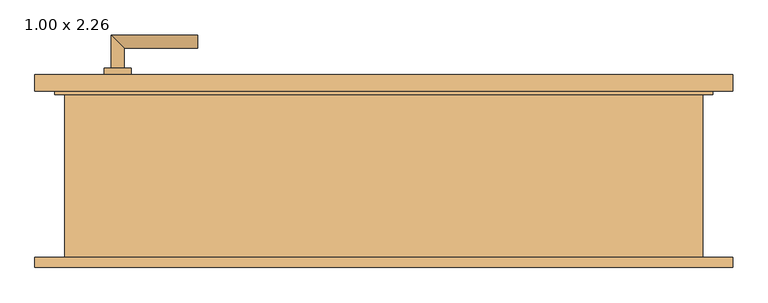
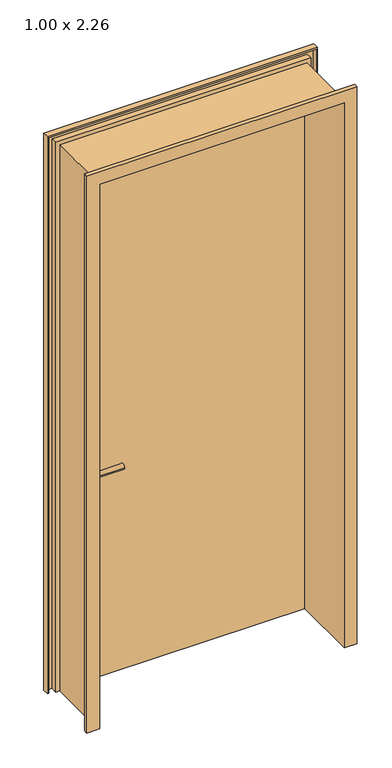
"""IFC4 building model written with IfcOpenShell, lengths in millimetres: door geometry, Drehflügel 1-flg - Stahlzarge : 1.00 x 2.26."""

import ifcopenshell
import ifcopenshell.guid

model = None  # the IFC model being written
_history = None  # IfcOwnerHistory: only IFC2X3 demands one
_inside = {}  # id of a spatial element -> (the spatial element, [elements in it])
_under = {}  # id of a project, library or spatial element -> (it, [spatial elements below it])
_declared = {}  # id of a project -> (the project, [libraries it declares])
_typed = {}  # id of a type object -> (the type object, [elements of that type])
_made_of = {}  # id of a material, layer set ... -> (it, [elements and type objects made of it])


def new_model(schema):
    """Start an empty IFC model of exactly this schema.

    Asked for "IFC4X3", IfcOpenShell would pick the latest addendum, in which some entities
    have other attributes; the version numbers below select the first issue.
    IFC2X3 requires an IfcOwnerHistory on every rooted entity: one is made here for all.
    """
    global model, _history
    if schema == "IFC4X3":
        model = ifcopenshell.file(schema_version=(4, 3, 0, 0))
    else:
        model = ifcopenshell.file(schema=schema)
    _inside.clear()
    _under.clear()
    _declared.clear()
    _typed.clear()
    _made_of.clear()
    _history = None
    if model.schema == "IFC2X3":
        org = make("IfcOrganization", Name="unknown")
        user = make(
            "IfcPersonAndOrganization",
            ThePerson=make("IfcPerson", FamilyName="unknown"),
            TheOrganization=org,
        )
        app = make(
            "IfcApplication",
            ApplicationDeveloper=org,
            Version="unknown",
            ApplicationFullName="unknown",
            ApplicationIdentifier="unknown",
        )
        _history = make(
            "IfcOwnerHistory",
            OwningUser=user,
            OwningApplication=app,
            ChangeAction="ADDED",
            CreationDate=0,
        )
    return model


def make(cls, **values):
    """One entity of the class cls with the attributes given. An attribute that is None is left unset."""
    return model.create_entity(
        cls, **{name: value for name, value in values.items() if value is not None}
    )


def rooted(cls, **values):
    """An entity with a GlobalId (a new one), such as an element, a storey or a relation."""
    return make(cls, GlobalId=ifcopenshell.guid.new(), OwnerHistory=_history, **values)


def si_unit(unit_type, name, prefix=None):
    """IfcSIUnit, for example si_unit("LENGTHUNIT", "METRE", prefix="MILLI")."""
    return make("IfcSIUnit", UnitType=unit_type, Prefix=prefix, Name=name)


def assignment(units):
    """IfcUnitAssignment: the units of a project."""
    return None if units is None else make("IfcUnitAssignment", Units=units)


def point(xyz):
    """IfcCartesianPoint."""
    return None if xyz is None else make("IfcCartesianPoint", Coordinates=xyz)


def direction(xyz):
    """IfcDirection."""
    return None if xyz is None else make("IfcDirection", DirectionRatios=xyz)


def frame(location, z_axis=None, x_axis=None):
    """IfcAxis2Placement3D, a coordinate frame: its origin and axes. An axis left out is left unset."""
    return make(
        "IfcAxis2Placement3D",
        Location=point(location),
        Axis=direction(z_axis),
        RefDirection=direction(x_axis),
    )


def frame_2d(location, x_axis=None):
    """IfcAxis2Placement2D, a coordinate frame in the plane: its origin and x axis."""
    return make(
        "IfcAxis2Placement2D", Location=point(location), RefDirection=direction(x_axis)
    )


def origin():
    """The frame at (0, 0, 0) with its axes left unset."""
    return frame((0.0, 0.0, 0.0))


def place(relative_to, where):
    """IfcLocalPlacement: puts the frame where relative to a parent placement (None: the world)."""
    return make(
        "IfcLocalPlacement", PlacementRelTo=relative_to, RelativePlacement=where
    )


def context(
    kind, dimensions, precision=None, world=None, true_north=None, identifier=None
):
    """IfcGeometricRepresentationContext, for example the 3D "Model" context."""
    return make(
        "IfcGeometricRepresentationContext",
        ContextIdentifier=identifier,
        ContextType=kind,
        CoordinateSpaceDimension=dimensions,
        Precision=precision,
        WorldCoordinateSystem=world,
        TrueNorth=true_north,
    )


def project(units=None, contexts=None):
    """IfcProject with its units and contexts."""
    return rooted(
        "IfcProject",
        Name="project",
        RepresentationContexts=contexts,
        UnitsInContext=assignment(units),
    )


def spatial(cls, under=None, at=None, **own):
    """A site, building, storey or space (cls), placed at a placement, below another one or the project."""
    s = rooted(cls, ObjectPlacement=at, **own)
    if under is not None:
        _under.setdefault(under.id(), (under, []))[1].append(s)
    return s


def polyline(points):
    """IfcPolyline through the points."""
    return make("IfcPolyline", Points=[point(p) for p in points])


def circle_curve(where, radius):
    """IfcCircle in the frame where."""
    return make("IfcCircle", Position=where, Radius=radius)


def ellipse_curve(where, semi_axis1, semi_axis2):
    """IfcEllipse in the frame where."""
    return make(
        "IfcEllipse", Position=where, SemiAxis1=semi_axis1, SemiAxis2=semi_axis2
    )


def trimmed(basis, trim1, trim2, sense, master):
    """IfcTrimmedCurve: the piece of a basis curve between two trims."""
    return make(
        "IfcTrimmedCurve",
        BasisCurve=basis,
        Trim1=trim1,
        Trim2=trim2,
        SenseAgreement=sense,
        MasterRepresentation=master,
    )


def segment(curve, same_sense, transition):
    """IfcCompositeCurveSegment."""
    return make(
        "IfcCompositeCurveSegment",
        Transition=transition,
        SameSense=same_sense,
        ParentCurve=curve,
    )


def composite_curve(segments, self_intersect=None):
    """IfcCompositeCurve: segments joined end to end."""
    return make("IfcCompositeCurve", Segments=segments, SelfIntersect=self_intersect)


def outline(outer, holes=None, kind="AREA"):
    """IfcArbitraryClosedProfileDef: a profile drawn as a closed curve; with holes, ...WithVoids."""
    if holes is None:
        return make("IfcArbitraryClosedProfileDef", ProfileType=kind, OuterCurve=outer)
    return make(
        "IfcArbitraryProfileDefWithVoids",
        ProfileType=kind,
        OuterCurve=outer,
        InnerCurves=holes,
    )


def extrude(swept, where, along, depth):
    """IfcExtrudedAreaSolid: the profile swept, set in the frame where, extruded along a direction by depth."""
    return make(
        "IfcExtrudedAreaSolid",
        SweptArea=swept,
        Position=where,
        ExtrudedDirection=direction(along),
        Depth=depth,
    )


def faces_of(points, faces, orient=None, outer=None):
    """IfcFace entities. A face is a list of loops; a loop is a list of indices into points, from 0.

    orient and outer hold one flag for each loop. By default every Orientation is true, the
    first loop of a face is its IfcFaceOuterBound and the others are IfcFaceBound.
    """
    made = []
    for i, loops in enumerate(faces):
        bounds = []
        for j, loop in enumerate(loops):
            is_outer = j == 0 if outer is None else outer[i][j]
            bounds.append(
                make(
                    "IfcFaceOuterBound" if is_outer else "IfcFaceBound",
                    Bound=make("IfcPolyLoop", Polygon=[points[k] for k in loop]),
                    Orientation=True if orient is None else orient[i][j],
                )
            )
        made.append(make("IfcFace", Bounds=bounds))
    return made


def faceted_brep(points, faces, orient=None, outer=None, voids=None):
    """IfcFacetedBrep: a solid bounded by flat faces; with voids (closed shells), ...WithVoids."""
    shared = [point(p) for p in points]
    hull = make("IfcClosedShell", CfsFaces=faces_of(shared, faces, orient, outer))
    if voids is None:
        return make("IfcFacetedBrep", Outer=hull)
    return make(
        "IfcFacetedBrepWithVoids",
        Outer=hull,
        Voids=[
            make(cls, CfsFaces=faces_of(shared, fs, o, b)) for cls, fs, o, b in voids
        ],
    )


def shape(context_of_items, identifier, shape_type, items):
    """IfcShapeRepresentation: the items that make up one representation, for example the "Body"."""
    return make(
        "IfcShapeRepresentation",
        ContextOfItems=context_of_items,
        RepresentationIdentifier=identifier,
        RepresentationType=shape_type,
        Items=items,
    )


def source(mapping_origin, context_of_items, identifier, shape_type, items):
    """IfcRepresentationMap: a shape defined once, which mapped items show again and again."""
    return make(
        "IfcRepresentationMap",
        MappingOrigin=mapping_origin,
        MappedRepresentation=shape(context_of_items, identifier, shape_type, items),
    )


def transform(
    local_origin,
    x_axis=None,
    y_axis=None,
    z_axis=None,
    scale=None,
    scale2=None,
    scale3=None,
    uniform=True,
):
    """IfcCartesianTransformationOperator3D, or its non-uniform kind. x_axis, y_axis, z_axis: its Axis1, 2, 3."""
    if uniform:
        return make(
            "IfcCartesianTransformationOperator3D",
            Axis1=direction(x_axis),
            Axis2=direction(y_axis),
            LocalOrigin=point(local_origin),
            Scale=scale,
            Axis3=direction(z_axis),
        )
    return make(
        "IfcCartesianTransformationOperator3DnonUniform",
        Axis1=direction(x_axis),
        Axis2=direction(y_axis),
        LocalOrigin=point(local_origin),
        Scale=scale,
        Axis3=direction(z_axis),
        Scale2=scale2,
        Scale3=scale3,
    )


def mapped(mapping_source, mapping_target):
    """IfcMappedItem: shows the shape of a source again, moved by a transform."""
    return make(
        "IfcMappedItem", MappingSource=mapping_source, MappingTarget=mapping_target
    )


def made_of(thing, what):
    """Note that an element or type object is made of a material, layer set ...; save() writes the relation."""
    if what is not None:
        _made_of.setdefault(what.id(), (what, []))[1].append(thing)
    return thing


def element(
    cls,
    number,
    at=None,
    inside=None,
    cuts=None,
    type_object=None,
    material=None,
    context=None,
    identifier="Body",
    shape_type=None,
    held_by="IfcProductDefinitionShape",
    body=None,
    shapes=None,
    **own,
):
    """One element of the class cls, such as IfcWall. Its Tag is "e" and its number.

    at: its placement. inside: the storey or other place that contains it. cuts: it is an
    opening in that element (IfcRelVoidsElement). A single representation is given by context,
    identifier, shape_type and body (its items); several are given by shapes. held_by: the class
    of the entity that holds the representations. save() writes the other relations.
    """
    e = rooted(cls, Tag="e%d" % number, ObjectPlacement=at, **own)
    if body is not None:
        shapes = [shape(context, identifier, shape_type, body)]
    if shapes is not None:
        e.Representation = make(held_by, Representations=shapes)
    if inside is not None:
        _inside.setdefault(inside.id(), (inside, []))[1].append(e)
    if cuts is not None:
        rooted(
            "IfcRelVoidsElement", RelatingBuildingElement=cuts, RelatedOpeningElement=e
        )
    if type_object is not None:
        _typed.setdefault(type_object.id(), (type_object, []))[1].append(e)
    return made_of(e, material)


def aggregate(whole, parts):
    """IfcRelAggregates: a whole, such as a stair, and the parts it consists of."""
    return rooted("IfcRelAggregates", RelatingObject=whole, RelatedObjects=parts)


def save(model, path):
    """Write the relations noted so far, then the file.

    IfcRelAggregates (storeys below a building ...), IfcRelContainedInSpatialStructure (elements
    in a storey), IfcRelDefinesByType, IfcRelAssociatesMaterial and IfcRelDeclares: one each for
    every whole, place, type object, material and project.
    """
    for whole, parts in _under.values():
        aggregate(whole, parts)
    for where, things in _inside.values():
        rooted(
            "IfcRelContainedInSpatialStructure",
            RelatedElements=things,
            RelatingStructure=where,
        )
    for kind, things in _typed.values():
        rooted("IfcRelDefinesByType", RelatedObjects=things, RelatingType=kind)
    for what, things in _made_of.values():
        rooted("IfcRelAssociatesMaterial", RelatedObjects=things, RelatingMaterial=what)
    for by, libraries in _declared.values():
        rooted("IfcRelDeclares", RelatingContext=by, RelatedDefinitions=libraries)
    model.write(path)


def plane_surface(at):
    """IfcPlane: the flat surface through the origin of the frame at, square to its z axis."""
    return make("IfcPlane", Position=at)


def cylinder_surface(at, radius):
    """IfcCylindricalSurface: all points at the distance radius from the z axis of the frame at."""
    return make("IfcCylindricalSurface", Position=at, Radius=radius)


def advanced_brep(points, edges, surfaces, faces):
    """IfcAdvancedBrep: a solid bounded by faces that lie on surfaces and meet in shared edges.

    An edge is (start, end): straight between two places in points (the first is 0);
    or (start, end, curve); or (start, end, curve, False) where it runs against its curve.
    A face is (place in surfaces, loops), or (place, loops, False) where it looks against
    its surface's normal. A loop lists edges by number (the first is 1), with a minus sign
    where the edge is run from its end to its start. The first loop is the outer one.
    """
    corners = [point(p) for p in points]
    vertices = [make("IfcVertexPoint", VertexGeometry=c) for c in corners]
    made = []
    for start, end, *more in edges:
        made.append(
            make(
                "IfcEdgeCurve",
                EdgeStart=vertices[start],
                EdgeEnd=vertices[end],
                EdgeGeometry=more[0] if more else make("IfcPolyline", Points=[corners[start], corners[end]]),
                SameSense=more[1] if len(more) > 1 else True,
            )
        )
    hull = []
    for where, loops, *sense in faces:
        bounds = []
        for j, loop in enumerate(loops):
            ring = [make("IfcOrientedEdge", EdgeElement=made[abs(k) - 1], Orientation=k > 0) for k in loop]
            bounds.append(
                make(
                    "IfcFaceOuterBound" if j == 0 else "IfcFaceBound",
                    Bound=make("IfcEdgeLoop", EdgeList=ring),
                    Orientation=True,
                )
            )
        hull.append(make("IfcAdvancedFace", Bounds=bounds, FaceSurface=surfaces[where], SameSense=sense[0] if sense else True))
    return make("IfcAdvancedBrep", Outer=make("IfcClosedShell", CfsFaces=hull))


def door_1_00_x_2_26_b1a9d28e(model_context):
    return source(origin(), model_context, "Body", "SolidModel", [
        advanced_brep(
        [(-410.0, 114.4346141, 1000.0), (-390.0, 114.4346141, 1000.0), (-410.0, 44.4346141, 1000.0), (-390.0, 64.4346141, 1000.0), (-280.0, 44.4346141, 1000.0), (-280.0, 64.4346141, 1000.0)],
        [
            (0, 1, circle_curve(frame((-400.0, 114.4346141, 1000.0), z_axis=(0.0, 1.0, 0.0), x_axis=(1.0, 0.0, 0.0)), 10.0)),
            (1, 0, circle_curve(frame((-400.0, 114.4346141, 1000.0), z_axis=(0.0, 1.0, 0.0), x_axis=(1.0, 0.0, 0.0)), 10.0)),
            (0, 2),
            (2, 3, ellipse_curve(frame((-400.0, 54.4346141, 1000.0), z_axis=(-0.7071067811865385, 0.7071067811865565, 0.0), x_axis=(0.7071067811865563, 0.7071067811865386, 0.0)), 14.1421356, 10.0)),
            (3, 1),
            (3, 2, ellipse_curve(frame((-400.0, 54.4346141, 1000.0), z_axis=(-0.7071067811865385, 0.7071067811865565, 0.0), x_axis=(0.7071067811865563, 0.7071067811865386, 0.0)), 14.1421356, 10.0)),
            (4, 5, circle_curve(frame((-280.0, 54.4346141, 1000.0), z_axis=(1.0, 0.0, 0.0), x_axis=(0.0, 1.0, 0.0)), 10.0)),
            (5, 4, circle_curve(frame((-280.0, 54.4346141, 1000.0), z_axis=(1.0, 0.0, 0.0), x_axis=(0.0, 1.0, 0.0)), 10.0)),
            (2, 4),
            (5, 3),
        ],
        [
            plane_surface(frame((-400.0, 114.4346141, -287.7526403), z_axis=(0.0, 1.0, 0.0), x_axis=(0.0, 0.0, 1.0))),
            cylinder_surface(frame((-400.0, 114.4346141, 1000.0), z_axis=(0.0, 1.0, 0.0), x_axis=(1.0, 0.0, 0.0)), 10.0),
            plane_surface(frame((-280.0, 54.4346141, -287.7526403), z_axis=(1.0, 0.0, 0.0), x_axis=(0.0, 0.0, 1.0))),
            cylinder_surface(frame((-400.0, 54.4346141, 1000.0), z_axis=(-1.0, 0.0, 0.0), x_axis=(0.0, 1.0, 0.0)), 10.0),
        ],
        [
            (0, [[1, 2]]),
            (1, [[-1, 3, 4, 5]]),
            (1, [[-2, -5, 6, -3]]),
            (2, [[7, 8]]),
            (3, [[-4, 9, -8, 10]]),
            (3, [[-6, -10, -7, -9]]),
        ],
    ),
        advanced_brep(
        [(-390.0, 174.4346141, 1000.0), (-410.0, 174.4346141, 1000.0), (-390.0, 204.4346141, 1000.0), (-410.0, 224.4346141, 1000.0), (-280.0, 204.4346141, 1000.0), (-280.0, 224.4346141, 1000.0)],
        [
            (0, 1, circle_curve(frame((-400.0, 174.4346141, 1000.0), z_axis=(0.0, -1.0, 0.0), x_axis=(-1.0, 0.0, 0.0)), 10.0)),
            (1, 0, circle_curve(frame((-400.0, 174.4346141, 1000.0), z_axis=(0.0, -1.0, 0.0), x_axis=(-1.0, 0.0, 0.0)), 10.0)),
            (0, 2),
            (2, 3, ellipse_curve(frame((-400.0, 214.4346141, 1000.0), z_axis=(-0.7071067811865475, -0.7071067811865475, 0.0), x_axis=(0.7071067811865474, -0.7071067811865476, 0.0)), 14.1421356, 10.0)),
            (3, 1),
            (3, 2, ellipse_curve(frame((-400.0, 214.4346141, 1000.0), z_axis=(-0.7071067811865475, -0.7071067811865475, 0.0), x_axis=(0.7071067811865474, -0.7071067811865476, 0.0)), 14.1421356, 10.0)),
            (4, 5, circle_curve(frame((-280.0, 214.4346141, 1000.0), z_axis=(1.0, 0.0, 0.0), x_axis=(0.0, 1.0, 0.0)), 10.0)),
            (5, 4, circle_curve(frame((-280.0, 214.4346141, 1000.0), z_axis=(1.0, 0.0, 0.0), x_axis=(0.0, 1.0, 0.0)), 10.0)),
            (2, 4),
            (5, 3),
        ],
        [
            plane_surface(frame((-400.0, 174.4346141, -287.7526403), z_axis=(0.0, -1.0, 0.0), x_axis=(0.0, 0.0, 1.0))),
            cylinder_surface(frame((-400.0, 174.4346141, 1000.0), z_axis=(0.0, -1.0, 0.0), x_axis=(-1.0, 0.0, 0.0)), 10.0),
            plane_surface(frame((-280.0, 214.4346141, -287.7526403), z_axis=(1.0, 0.0, 0.0), x_axis=(0.0, 0.0, 1.0))),
            cylinder_surface(frame((-400.0, 214.4346141, 1000.0), z_axis=(-1.0, 0.0, 0.0), x_axis=(0.0, 1.0, 0.0)), 10.0),
        ],
        [
            (0, [[1, 2]]),
            (1, [[-1, 3, 4, 5]]),
            (1, [[-2, -5, 6, -3]]),
            (2, [[7, 8]]),
            (3, [[-4, 9, -8, 10]]),
            (3, [[-6, -10, -7, -9]]),
        ],
    ),
        extrude(outline(composite_curve([segment(trimmed(circle_curve(frame_2d((1000.0, -400.0)), 20.0), [point((1000.0, -420.0))], [point((1000.0, -380.0))], False, "CARTESIAN"), True, "CONTINUOUS"), segment(trimmed(circle_curve(frame_2d((1000.0, -400.0)), 20.0), [point((1000.0, -380.0))], [point((1000.0, -420.0))], False, "CARTESIAN"), True, "CONTINUOUS")], self_intersect=False)), frame((0.0, 104.4346141, 0.0), z_axis=(0.0, 1.0, 0.0), x_axis=(0.0, 0.0, 1.0)), (0.0, 0.0, 1.0), 10.0),
        extrude(outline(composite_curve([segment(trimmed(circle_curve(frame_2d((1000.0, -400.0)), 20.0), [point((1000.0, -420.0))], [point((1000.0, -380.0))], False, "CARTESIAN"), True, "CONTINUOUS"), segment(trimmed(circle_curve(frame_2d((1000.0, -400.0)), 20.0), [point((1000.0, -380.0))], [point((1000.0, -420.0))], False, "CARTESIAN"), True, "CONTINUOUS")], self_intersect=False)), frame((0.0, 164.4346141, 0.0), z_axis=(0.0, 1.0, 0.0), x_axis=(0.0, 0.0, 1.0)), (0.0, 0.0, 1.0), 10.0),
        extrude(outline(polyline([(490.0, 139.4346141), (-490.0, 139.4346141), (-490.0, 164.4346141), (490.0, 164.4346141), (490.0, 139.4346141)])), frame((0.0, 0.0, 100.0), z_axis=(0.0, 0.0, 1.0), x_axis=(1.0, 0.0, 0.0)), (0.0, 0.0, 1.0), 2250.0),
        faceted_brep([(524.4603207, -125.5653859, 100.0), (475.0, -125.5653859, 100.0), (475.0, 139.4346141, 100.0), (490.0, 139.4346141, 100.0), (490.0, 164.4346141, 100.0), (524.4603207, 164.4346141, 100.0), (524.4603207, 139.4346141, 100.0), (519.4603207, 139.4346141, 100.0), (519.4603207, 159.4346141, 100.0), (495.0, 159.4346141, 100.0), (495.0, 134.4346141, 100.0), (480.0, 134.4346141, 100.0), (480.0, -120.5653859, 100.0), (519.4603207, -120.5653859, 100.0), (519.4603207, -110.5653859, 100.0), (524.4603207, -110.5653859, 100.0), (524.4603207, -125.5653859, 2384.4603207), (-524.4603207, -125.5653859, 2384.4603207), (-524.4603207, -125.5653859, 100.0), (-475.0, -125.5653859, 100.0), (-475.0, -125.5653859, 2335.0), (475.0, -125.5653859, 2335.0), (475.0, 139.4346141, 2335.0), (-475.0, 139.4346141, 2335.0), (-475.0, 139.4346141, 100.0), (-490.0, 139.4346141, 100.0), (-490.0, 139.4346141, 2350.0), (490.0, 139.4346141, 2350.0), (490.0, 164.4346141, 2350.0), (-490.0, 164.4346141, 2350.0), (-490.0, 164.4346141, 100.0), (-524.4603207, 164.4346141, 100.0), (-524.4603207, 164.4346141, 2384.4603207), (524.4603207, 164.4346141, 2384.4603207), (524.4603207, 139.4346141, 2384.4603207), (-524.4603207, 139.4346141, 2384.4603207), (-524.4603207, 139.4346141, 100.0), (-519.4603207, 139.4346141, 100.0), (-519.4603207, 139.4346141, 2379.4603207), (519.4603207, 139.4346141, 2379.4603207), (519.4603207, 159.4346141, 2379.4603207), (-519.4603207, 159.4346141, 2379.4603207), (-519.4603207, 159.4346141, 100.0), (-495.0, 159.4346141, 100.0), (-495.0, 159.4346141, 2355.0), (495.0, 159.4346141, 2355.0), (495.0, 134.4346141, 2355.0), (-495.0, 134.4346141, 2355.0), (-495.0, 134.4346141, 100.0), (-480.0, 134.4346141, 100.0), (-480.0, 134.4346141, 2340.0), (480.0, 134.4346141, 2340.0), (480.0, -120.5653859, 2340.0), (-480.0, -120.5653859, 2340.0), (-480.0, -120.5653859, 100.0), (-519.4603207, -120.5653859, 100.0), (-519.4603207, -120.5653859, 2379.4603207), (519.4603207, -120.5653859, 2379.4603207), (519.4603207, -110.5653859, 2379.4603207), (-519.4603207, -110.5653859, 2379.4603207), (-519.4603207, -110.5653859, 100.0), (-524.4603207, -110.5653859, 100.0), (-524.4603207, -110.5653859, 2384.4603207), (524.4603207, -110.5653859, 2384.4603207)], [[[0, 1, 2, 3, 4, 5, 6, 7, 8, 9, 10, 11, 12, 13, 14, 15]], [[1, 0, 16, 17, 18, 19, 20, 21]], [[2, 1, 21, 22]], [[3, 2, 22, 23, 24, 25, 26, 27]], [[4, 3, 27, 28]], [[5, 4, 28, 29, 30, 31, 32, 33]], [[6, 5, 33, 34]], [[7, 6, 34, 35, 36, 37, 38, 39]], [[8, 7, 39, 40]], [[9, 8, 40, 41, 42, 43, 44, 45]], [[10, 9, 45, 46]], [[11, 10, 46, 47, 48, 49, 50, 51]], [[12, 11, 51, 52]], [[13, 12, 52, 53, 54, 55, 56, 57]], [[14, 13, 57, 58]], [[15, 14, 58, 59, 60, 61, 62, 63]], [[0, 15, 63, 16]], [[17, 62, 61, 18]], [[18, 61, 60, 55, 54, 49, 48, 43, 42, 37, 36, 31, 30, 25, 24, 19]], [[23, 20, 19, 24]], [[29, 26, 25, 30]], [[35, 32, 31, 36]], [[41, 38, 37, 42]], [[47, 44, 43, 48]], [[53, 50, 49, 54]], [[59, 56, 55, 60]], [[22, 21, 20, 23]], [[28, 27, 26, 29]], [[34, 33, 32, 35]], [[40, 39, 38, 41]], [[46, 45, 44, 47]], [[52, 51, 50, 53]], [[58, 57, 56, 59]], [[16, 63, 62, 17]]]),
    ])


if __name__ == "__main__":
    model = new_model("IFC4")
    model_context = context("Model", 3, world=origin())
    ifc_project = project(units=[si_unit("LENGTHUNIT", "METRE", prefix="MILLI")], contexts=[model_context])
    site = spatial("IfcSite", under=ifc_project)
    building = spatial("IfcBuilding", under=site)
    placement = place(None, origin())
    door_1_00_x_2_26_shape = door_1_00_x_2_26_b1a9d28e(model_context)
    element("IfcDoor", 1, ObjectType="Drehflügel 1-flg - Stahlzarge : 1.00 x 2.26", at=placement, inside=building, context=model_context, shape_type="MappedRepresentation", body=[
        mapped(door_1_00_x_2_26_shape, transform((0.0, 0.0, 0.0), x_axis=(1.0, 0.0, 0.0), y_axis=(0.0, 1.0, 0.0), z_axis=(0.0, 0.0, 1.0))),
    ])
    save(model, "model.ifc")

# Revit data of these elements
# Type "Drehflügel 1-flg - Stahlzarge : 1.00 x 2.26"
#   Construction Type Id = "MDOOR"
#   Type Mark = "20"
#   Operation = "SingleSwingRight"
#   Keynote = "16.03"
#   Analytic Construction = "Metall"
#   Thermal Resistance (R) = 0.270117 (m²·K)/W
#   Heat Transfer Coefficient (U) = 3.7021 W/(m²·K)
#   Rough Width = 1.000 m
#   Rough Height [instance default] = 2.360 m
#   Höhe Türgriff [instance default] = 0.900 m
#   Height = 2.260 m
#   Fußbodenaufbau [instance default] = 0.100 m
#   Width = 1.000 m
#   Sichtbarkeit Sturzlinien [instance default] = yes
#   Türgriff auswählen [instance default] = element 221079
#   Türgriff [instance default] = none
#   Türflügel [instance default] = none
#   Rahmen/Pfosten [instance default] = Metall - Lackiert - Grau
#   Visual Light Transmittance = 0
#   Solar Heat Gain Coefficient = 0
#   Function = (empty or 0)
#   Wall Closure = (empty or 0)
# Element 1 (IfcDoor, "Drehflügel 1-flg - Stahlzarge : 1.00 x 2.26")
#   Materials on its faces: "Metall - Lackiert - Grau", "Metall - Chrom", "Holz - Birke"
# Materials
#   "Metall - Lackiert - Grau": class "Farbe 1", colour RGB 98 98 98, transparency 0, Cost = 0
#   "Metall - Chrom": class "Metall", colour RGB 247 247 247, transparency 0, Cost = 0
#   "Holz - Birke": class "Holz", colour RGB 213 164 103, transparency 0, Cost = 0
